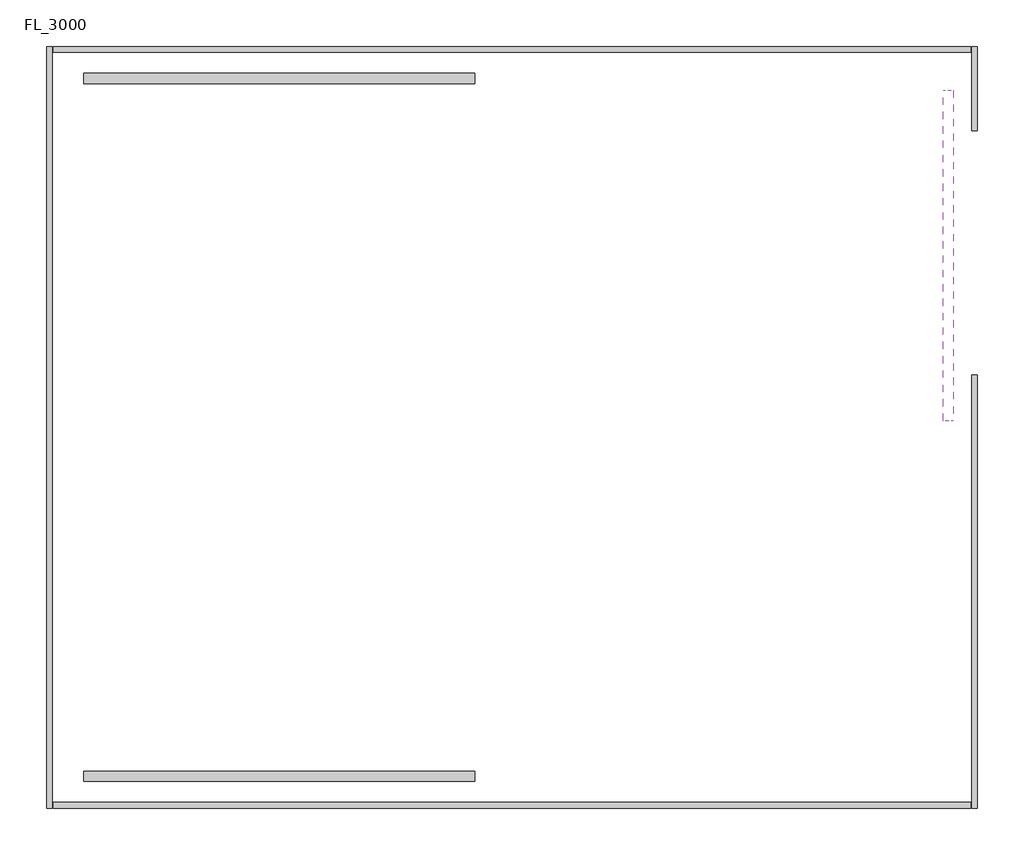
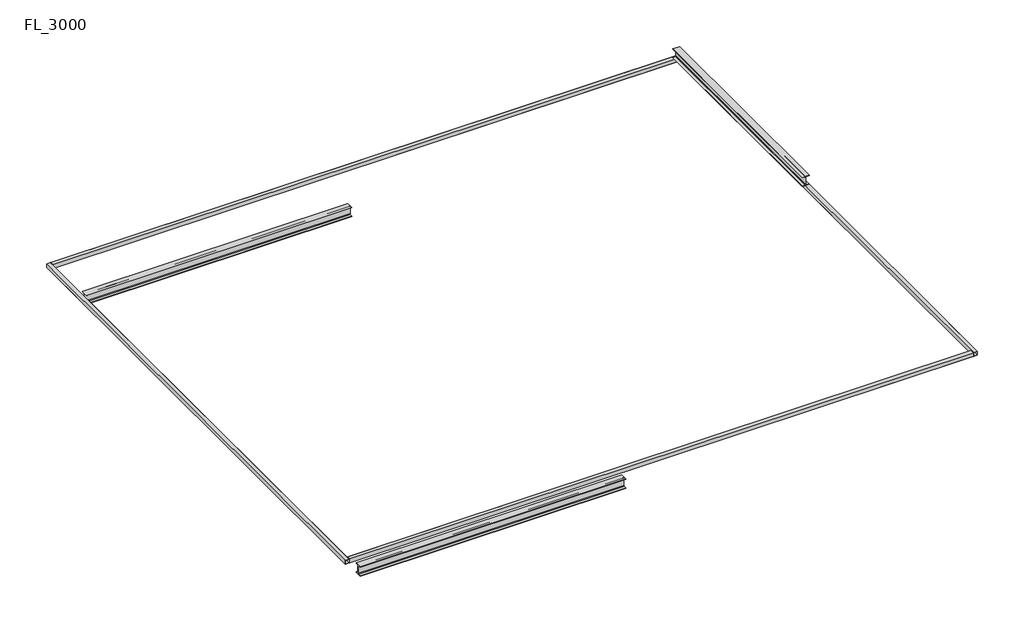
# One storey: 8 beams.
"""IFC4 building model written with IfcOpenShell, lengths in millimetres."""

import ifcopenshell
import ifcopenshell.guid

model = None  # the IFC model being written
_history = None  # IfcOwnerHistory: only IFC2X3 demands one
_inside = {}  # id of a spatial element -> (the spatial element, [elements in it])
_under = {}  # id of a project, library or spatial element -> (it, [spatial elements below it])
_declared = {}  # id of a project -> (the project, [libraries it declares])
_typed = {}  # id of a type object -> (the type object, [elements of that type])
_made_of = {}  # id of a material, layer set ... -> (it, [elements and type objects made of it])


def new_model(schema):
    """Start an empty IFC model of exactly this schema.

    Asked for "IFC4X3", IfcOpenShell would pick the latest addendum, in which some entities
    have other attributes; the version numbers below select the first issue.
    IFC2X3 requires an IfcOwnerHistory on every rooted entity: one is made here for all.
    """
    global model, _history
    if schema == "IFC4X3":
        model = ifcopenshell.file(schema_version=(4, 3, 0, 0))
    else:
        model = ifcopenshell.file(schema=schema)
    _inside.clear()
    _under.clear()
    _declared.clear()
    _typed.clear()
    _made_of.clear()
    _history = None
    if model.schema == "IFC2X3":
        org = make("IfcOrganization", Name="unknown")
        user = make(
            "IfcPersonAndOrganization",
            ThePerson=make("IfcPerson", FamilyName="unknown"),
            TheOrganization=org,
        )
        app = make(
            "IfcApplication",
            ApplicationDeveloper=org,
            Version="unknown",
            ApplicationFullName="unknown",
            ApplicationIdentifier="unknown",
        )
        _history = make(
            "IfcOwnerHistory",
            OwningUser=user,
            OwningApplication=app,
            ChangeAction="ADDED",
            CreationDate=0,
        )
    return model


def make(cls, **values):
    """One entity of the class cls with the attributes given. An attribute that is None is left unset."""
    return model.create_entity(
        cls, **{name: value for name, value in values.items() if value is not None}
    )


def rooted(cls, **values):
    """An entity with a GlobalId (a new one), such as an element, a storey or a relation."""
    return make(cls, GlobalId=ifcopenshell.guid.new(), OwnerHistory=_history, **values)


def si_unit(unit_type, name, prefix=None):
    """IfcSIUnit, for example si_unit("LENGTHUNIT", "METRE", prefix="MILLI")."""
    return make("IfcSIUnit", UnitType=unit_type, Prefix=prefix, Name=name)


def assignment(units):
    """IfcUnitAssignment: the units of a project."""
    return None if units is None else make("IfcUnitAssignment", Units=units)


def point(xyz):
    """IfcCartesianPoint."""
    return None if xyz is None else make("IfcCartesianPoint", Coordinates=xyz)


def direction(xyz):
    """IfcDirection."""
    return None if xyz is None else make("IfcDirection", DirectionRatios=xyz)


def frame(location, z_axis=None, x_axis=None):
    """IfcAxis2Placement3D, a coordinate frame: its origin and axes. An axis left out is left unset."""
    return make(
        "IfcAxis2Placement3D",
        Location=point(location),
        Axis=direction(z_axis),
        RefDirection=direction(x_axis),
    )


def frame_2d(location, x_axis=None):
    """IfcAxis2Placement2D, a coordinate frame in the plane: its origin and x axis."""
    return make(
        "IfcAxis2Placement2D", Location=point(location), RefDirection=direction(x_axis)
    )


def origin():
    """The frame at (0, 0, 0) with its axes left unset."""
    return frame((0.0, 0.0, 0.0))


def place(relative_to, where):
    """IfcLocalPlacement: puts the frame where relative to a parent placement (None: the world)."""
    return make(
        "IfcLocalPlacement", PlacementRelTo=relative_to, RelativePlacement=where
    )


def context(
    kind, dimensions, precision=None, world=None, true_north=None, identifier=None
):
    """IfcGeometricRepresentationContext, for example the 3D "Model" context."""
    return make(
        "IfcGeometricRepresentationContext",
        ContextIdentifier=identifier,
        ContextType=kind,
        CoordinateSpaceDimension=dimensions,
        Precision=precision,
        WorldCoordinateSystem=world,
        TrueNorth=true_north,
    )


def project(units=None, contexts=None):
    """IfcProject with its units and contexts."""
    return rooted(
        "IfcProject",
        Name="project",
        RepresentationContexts=contexts,
        UnitsInContext=assignment(units),
    )


def spatial(cls, under=None, at=None, **own):
    """A site, building, storey or space (cls), placed at a placement, below another one or the project."""
    s = rooted(cls, ObjectPlacement=at, **own)
    if under is not None:
        _under.setdefault(under.id(), (under, []))[1].append(s)
    return s


def polyline(points):
    """IfcPolyline through the points."""
    return make("IfcPolyline", Points=[point(p) for p in points])


def circle_curve(where, radius):
    """IfcCircle in the frame where."""
    return make("IfcCircle", Position=where, Radius=radius)


def trimmed(basis, trim1, trim2, sense, master):
    """IfcTrimmedCurve: the piece of a basis curve between two trims."""
    return make(
        "IfcTrimmedCurve",
        BasisCurve=basis,
        Trim1=trim1,
        Trim2=trim2,
        SenseAgreement=sense,
        MasterRepresentation=master,
    )


def segment(curve, same_sense, transition):
    """IfcCompositeCurveSegment."""
    return make(
        "IfcCompositeCurveSegment",
        Transition=transition,
        SameSense=same_sense,
        ParentCurve=curve,
    )


def composite_curve(segments, self_intersect=None):
    """IfcCompositeCurve: segments joined end to end."""
    return make("IfcCompositeCurve", Segments=segments, SelfIntersect=self_intersect)


def outline(outer, holes=None, kind="AREA"):
    """IfcArbitraryClosedProfileDef: a profile drawn as a closed curve; with holes, ...WithVoids."""
    if holes is None:
        return make("IfcArbitraryClosedProfileDef", ProfileType=kind, OuterCurve=outer)
    return make(
        "IfcArbitraryProfileDefWithVoids",
        ProfileType=kind,
        OuterCurve=outer,
        InnerCurves=holes,
    )


def extrude(swept, where, along, depth):
    """IfcExtrudedAreaSolid: the profile swept, set in the frame where, extruded along a direction by depth."""
    return make(
        "IfcExtrudedAreaSolid",
        SweptArea=swept,
        Position=where,
        ExtrudedDirection=direction(along),
        Depth=depth,
    )


def shape(context_of_items, identifier, shape_type, items):
    """IfcShapeRepresentation: the items that make up one representation, for example the "Body"."""
    return make(
        "IfcShapeRepresentation",
        ContextOfItems=context_of_items,
        RepresentationIdentifier=identifier,
        RepresentationType=shape_type,
        Items=items,
    )


def source(mapping_origin, context_of_items, identifier, shape_type, items):
    """IfcRepresentationMap: a shape defined once, which mapped items show again and again."""
    return make(
        "IfcRepresentationMap",
        MappingOrigin=mapping_origin,
        MappedRepresentation=shape(context_of_items, identifier, shape_type, items),
    )


def transform(
    local_origin,
    x_axis=None,
    y_axis=None,
    z_axis=None,
    scale=None,
    scale2=None,
    scale3=None,
    uniform=True,
):
    """IfcCartesianTransformationOperator3D, or its non-uniform kind. x_axis, y_axis, z_axis: its Axis1, 2, 3."""
    if uniform:
        return make(
            "IfcCartesianTransformationOperator3D",
            Axis1=direction(x_axis),
            Axis2=direction(y_axis),
            LocalOrigin=point(local_origin),
            Scale=scale,
            Axis3=direction(z_axis),
        )
    return make(
        "IfcCartesianTransformationOperator3DnonUniform",
        Axis1=direction(x_axis),
        Axis2=direction(y_axis),
        LocalOrigin=point(local_origin),
        Scale=scale,
        Axis3=direction(z_axis),
        Scale2=scale2,
        Scale3=scale3,
    )


def mapped(mapping_source, mapping_target):
    """IfcMappedItem: shows the shape of a source again, moved by a transform."""
    return make(
        "IfcMappedItem", MappingSource=mapping_source, MappingTarget=mapping_target
    )


def made_of(thing, what):
    """Note that an element or type object is made of a material, layer set ...; save() writes the relation."""
    if what is not None:
        _made_of.setdefault(what.id(), (what, []))[1].append(thing)
    return thing


def element(
    cls,
    number,
    at=None,
    inside=None,
    cuts=None,
    type_object=None,
    material=None,
    context=None,
    identifier="Body",
    shape_type=None,
    held_by="IfcProductDefinitionShape",
    body=None,
    shapes=None,
    **own,
):
    """One element of the class cls, such as IfcWall. Its Tag is "e" and its number.

    at: its placement. inside: the storey or other place that contains it. cuts: it is an
    opening in that element (IfcRelVoidsElement). A single representation is given by context,
    identifier, shape_type and body (its items); several are given by shapes. held_by: the class
    of the entity that holds the representations. save() writes the other relations.
    """
    e = rooted(cls, Tag="e%d" % number, ObjectPlacement=at, **own)
    if body is not None:
        shapes = [shape(context, identifier, shape_type, body)]
    if shapes is not None:
        e.Representation = make(held_by, Representations=shapes)
    if inside is not None:
        _inside.setdefault(inside.id(), (inside, []))[1].append(e)
    if cuts is not None:
        rooted(
            "IfcRelVoidsElement", RelatingBuildingElement=cuts, RelatedOpeningElement=e
        )
    if type_object is not None:
        _typed.setdefault(type_object.id(), (type_object, []))[1].append(e)
    return made_of(e, material)


def aggregate(whole, parts):
    """IfcRelAggregates: a whole, such as a stair, and the parts it consists of."""
    return rooted("IfcRelAggregates", RelatingObject=whole, RelatedObjects=parts)


def save(model, path):
    """Write the relations noted so far, then the file.

    IfcRelAggregates (storeys below a building ...), IfcRelContainedInSpatialStructure (elements
    in a storey), IfcRelDefinesByType, IfcRelAssociatesMaterial and IfcRelDeclares: one each for
    every whole, place, type object, material and project.
    """
    for whole, parts in _under.values():
        aggregate(whole, parts)
    for where, things in _inside.values():
        rooted(
            "IfcRelContainedInSpatialStructure",
            RelatedElements=things,
            RelatingStructure=where,
        )
    for kind, things in _typed.values():
        rooted("IfcRelDefinesByType", RelatedObjects=things, RelatingType=kind)
    for what, things in _made_of.values():
        rooted("IfcRelAssociatesMaterial", RelatedObjects=things, RelatingMaterial=what)
    for by, libraries in _declared.values():
        rooted("IfcRelDeclares", RelatingContext=by, RelatedDefinitions=libraries)
    model.write(path)


def steel_h_beam_22148b76(model_context):
    return source(origin(), model_context, "Body", "SweptSolid", [
        extrude(outline(composite_curve([segment(polyline([(87.5, -111.0), (87.5, -122.0), (-87.5, -122.0), (-87.5, -111.0), (-19.5, -111.0)]), True, "CONTINUOUS"), segment(trimmed(circle_curve(frame_2d((-19.5, -95.0)), 16.0), [point((-19.5, -111.0))], [point((-3.5, -95.0))], True, "CARTESIAN"), True, "CONTINUOUS"), segment(polyline([(-3.5, -95.0), (-3.5, 95.0)]), True, "CONTINUOUS"), segment(trimmed(circle_curve(frame_2d((-19.5, 95.0)), 16.0), [point((-3.5, 95.0))], [point((-19.5, 111.0))], True, "CARTESIAN"), True, "CONTINUOUS"), segment(polyline([(-19.5, 111.0), (-87.5, 111.0), (-87.5, 122.0), (87.5, 122.0), (87.5, 111.0), (19.5, 111.0)]), True, "CONTINUOUS"), segment(trimmed(circle_curve(frame_2d((19.5, 95.0)), 16.0), [point((19.5, 111.0))], [point((3.5, 95.0))], True, "CARTESIAN"), True, "CONTINUOUS"), segment(polyline([(3.5, 95.0), (3.5, -95.0)]), True, "CONTINUOUS"), segment(trimmed(circle_curve(frame_2d((19.5, -95.0)), 16.0), [point((3.5, -95.0))], [point((19.5, -111.0))], True, "CARTESIAN"), True, "CONTINUOUS"), segment(polyline([(19.5, -111.0), (87.5, -111.0)]), True, "CONTINUOUS")], self_intersect=False)), frame((-3361.8243373, 0.0, 0.0), z_axis=(1.0, 0.0, 0.0), x_axis=(0.0, 1.0, 0.0)), (0.0, 0.0, 1.0), 6724.6),
    ])


def steel_h_beam_0520d745(model_context):
    return source(origin(), model_context, "Body", "SweptSolid", [
        extrude(outline(composite_curve([segment(polyline([(87.5, -111.0), (87.5, -122.0), (-87.5, -122.0), (-87.5, -111.0), (-19.5, -111.0)]), True, "CONTINUOUS"), segment(trimmed(circle_curve(frame_2d((-19.5, -95.0)), 16.0), [point((-19.5, -111.0))], [point((-3.5, -95.0))], True, "CARTESIAN"), True, "CONTINUOUS"), segment(polyline([(-3.5, -95.0), (-3.5, 95.0)]), True, "CONTINUOUS"), segment(trimmed(circle_curve(frame_2d((-19.5, 95.0)), 16.0), [point((-3.5, 95.0))], [point((-19.5, 111.0))], True, "CARTESIAN"), True, "CONTINUOUS"), segment(polyline([(-19.5, 111.0), (-87.5, 111.0), (-87.5, 122.0), (87.5, 122.0), (87.5, 111.0), (19.5, 111.0)]), True, "CONTINUOUS"), segment(trimmed(circle_curve(frame_2d((19.5, 95.0)), 16.0), [point((19.5, 111.0))], [point((3.5, 95.0))], True, "CARTESIAN"), True, "CONTINUOUS"), segment(polyline([(3.5, 95.0), (3.5, -95.0)]), True, "CONTINUOUS"), segment(trimmed(circle_curve(frame_2d((19.5, -95.0)), 16.0), [point((3.5, -95.0))], [point((19.5, -111.0))], True, "CARTESIAN"), True, "CONTINUOUS"), segment(polyline([(19.5, -111.0), (87.5, -111.0)]), True, "CONTINUOUS")], self_intersect=False)), frame((-3363.2513255, 0.0, 0.0), z_axis=(1.0, 0.0, 0.0), x_axis=(0.0, 1.0, 0.0)), (0.0, 0.0, 1.0), 6724.6),
    ])


def steel_h_beam_2cee67ca(model_context):
    return source(origin(), model_context, "Body", "SweptSolid", [
        extrude(outline(composite_curve([segment(polyline([(87.5, -111.0), (87.5, -122.0), (-87.5, -122.0), (-87.5, -111.0), (-19.5, -111.0)]), True, "CONTINUOUS"), segment(trimmed(circle_curve(frame_2d((-19.5, -95.0)), 16.0), [point((-19.5, -111.0))], [point((-3.5, -95.0))], True, "CARTESIAN"), True, "CONTINUOUS"), segment(polyline([(-3.5, -95.0), (-3.5, 95.0)]), True, "CONTINUOUS"), segment(trimmed(circle_curve(frame_2d((-19.5, 95.0)), 16.0), [point((-3.5, 95.0))], [point((-19.5, 111.0))], True, "CARTESIAN"), True, "CONTINUOUS"), segment(polyline([(-19.5, 111.0), (-87.5, 111.0), (-87.5, 122.0), (87.5, 122.0), (87.5, 111.0), (19.5, 111.0)]), True, "CONTINUOUS"), segment(trimmed(circle_curve(frame_2d((19.5, 95.0)), 16.0), [point((19.5, 111.0))], [point((3.5, 95.0))], True, "CARTESIAN"), True, "CONTINUOUS"), segment(polyline([(3.5, 95.0), (3.5, -95.0)]), True, "CONTINUOUS"), segment(trimmed(circle_curve(frame_2d((19.5, -95.0)), 16.0), [point((3.5, -95.0))], [point((19.5, -111.0))], True, "CARTESIAN"), True, "CONTINUOUS"), segment(polyline([(19.5, -111.0), (87.5, -111.0)]), True, "CONTINUOUS")], self_intersect=False)), frame((-2886.3486745, 0.0, 0.0), z_axis=(1.0, 0.0, 0.0), x_axis=(0.0, 1.0, 0.0)), (0.0, 0.0, 1.0), 5681.8597388),
    ])


def steel_rectangular_beam_bm125_rt_100x100x4_0_fd47acba(model_context):
    return source(origin(), model_context, "Body", "SweptSolid", [
        extrude(outline(polyline([(-50.0, 50.0), (50.0, 50.0), (50.0, -50.0), (-50.0, -50.0), (-50.0, 50.0)]), holes=[polyline([(46.0, -46.0), (46.0, 46.0), (-46.0, 46.0), (-46.0, -46.0), (46.0, -46.0)])]), frame((-7887.3, 0.0, 0.0), z_axis=(1.0, 0.0, 0.0), x_axis=(0.0, 1.0, 0.0)), (0.0, 0.0, 1.0), 15774.6),
        extrude(outline(polyline([(-50.0, 50.0), (50.0, 50.0), (50.0, -50.0), (-50.0, -50.0), (-50.0, 50.0)]), holes=[polyline([(46.0, -46.0), (46.0, 46.0), (-46.0, 46.0), (-46.0, -46.0), (46.0, -46.0)])]), frame((-7887.3, 0.0, 0.0), z_axis=(1.0, 0.0, 0.0), x_axis=(0.0, 1.0, 0.0)), (0.0, 0.0, 1.0), 15774.6),
        extrude(outline(polyline([(-50.0, 50.0), (50.0, 50.0), (50.0, -50.0), (-50.0, -50.0), (-50.0, 50.0)]), holes=[polyline([(46.0, -46.0), (46.0, 46.0), (-46.0, 46.0), (-46.0, -46.0), (46.0, -46.0)])]), frame((-7887.3, 0.0, 0.0), z_axis=(1.0, 0.0, 0.0), x_axis=(0.0, 1.0, 0.0)), (0.0, 0.0, 1.0), 15774.6),
        extrude(outline(polyline([(-50.0, 50.0), (50.0, 50.0), (50.0, -50.0), (-50.0, -50.0), (-50.0, 50.0)]), holes=[polyline([(46.0, -46.0), (46.0, 46.0), (-46.0, 46.0), (-46.0, -46.0), (46.0, -46.0)])]), frame((-7887.3, 0.0, 0.0), z_axis=(1.0, 0.0, 0.0), x_axis=(0.0, 1.0, 0.0)), (0.0, 0.0, 1.0), 15774.6),
    ])


def steel_rectangular_beam_bm125_rt_100x100x4_0_2c93a6f0(model_context):
    return source(origin(), model_context, "Body", "SweptSolid", [
        extrude(outline(polyline([(-50.0, 50.0), (50.0, 50.0), (50.0, -50.0), (-50.0, -50.0), (-50.0, 50.0)]), holes=[polyline([(46.0, -46.0), (46.0, 46.0), (-46.0, 46.0), (-46.0, -46.0), (46.0, -46.0)])]), frame((-6550.0, 0.0, 0.0), z_axis=(1.0, 0.0, 0.0), x_axis=(0.0, 1.0, 0.0)), (0.0, 0.0, 1.0), 13100.0),
        extrude(outline(polyline([(-50.0, 50.0), (50.0, 50.0), (50.0, -50.0), (-50.0, -50.0), (-50.0, 50.0)]), holes=[polyline([(46.0, -46.0), (46.0, 46.0), (-46.0, 46.0), (-46.0, -46.0), (46.0, -46.0)])]), frame((-6550.0, 0.0, 0.0), z_axis=(1.0, 0.0, 0.0), x_axis=(0.0, 1.0, 0.0)), (0.0, 0.0, 1.0), 13100.0),
        extrude(outline(polyline([(-50.0, 50.0), (50.0, 50.0), (50.0, -50.0), (-50.0, -50.0), (-50.0, 50.0)]), holes=[polyline([(46.0, -46.0), (46.0, 46.0), (-46.0, 46.0), (-46.0, -46.0), (46.0, -46.0)])]), frame((-6550.0, 0.0, 0.0), z_axis=(1.0, 0.0, 0.0), x_axis=(0.0, 1.0, 0.0)), (0.0, 0.0, 1.0), 13100.0),
        extrude(outline(polyline([(-50.0, 50.0), (50.0, 50.0), (50.0, -50.0), (-50.0, -50.0), (-50.0, 50.0)]), holes=[polyline([(46.0, -46.0), (46.0, 46.0), (-46.0, 46.0), (-46.0, -46.0), (46.0, -46.0)])]), frame((-6550.0, 0.0, 0.0), z_axis=(1.0, 0.0, 0.0), x_axis=(0.0, 1.0, 0.0)), (0.0, 0.0, 1.0), 13100.0),
    ])


def steel_rectangular_beam_bm125_rt_100x100x4_0_60a5dd41(model_context):
    return source(origin(), model_context, "Body", "SweptSolid", [
        extrude(outline(polyline([(-50.0, 50.0), (50.0, 50.0), (50.0, -50.0), (-50.0, -50.0), (-50.0, 50.0)]), holes=[polyline([(46.0, -46.0), (46.0, 46.0), (-46.0, 46.0), (-46.0, -46.0), (46.0, -46.0)])]), frame((-3725.0, 0.0, 0.0), z_axis=(1.0, 0.0, 0.0), x_axis=(0.0, 1.0, 0.0)), (0.0, 0.0, 1.0), 7450.0),
        extrude(outline(polyline([(-50.0, 50.0), (50.0, 50.0), (50.0, -50.0), (-50.0, -50.0), (-50.0, 50.0)]), holes=[polyline([(46.0, -46.0), (46.0, 46.0), (-46.0, 46.0), (-46.0, -46.0), (46.0, -46.0)])]), frame((-3725.0, 0.0, 0.0), z_axis=(1.0, 0.0, 0.0), x_axis=(0.0, 1.0, 0.0)), (0.0, 0.0, 1.0), 7450.0),
        extrude(outline(polyline([(-50.0, 50.0), (50.0, 50.0), (50.0, -50.0), (-50.0, -50.0), (-50.0, 50.0)]), holes=[polyline([(46.0, -46.0), (46.0, 46.0), (-46.0, 46.0), (-46.0, -46.0), (46.0, -46.0)])]), frame((-3725.0, 0.0, 0.0), z_axis=(1.0, 0.0, 0.0), x_axis=(0.0, 1.0, 0.0)), (0.0, 0.0, 1.0), 7450.0),
        extrude(outline(polyline([(-50.0, 50.0), (50.0, 50.0), (50.0, -50.0), (-50.0, -50.0), (-50.0, 50.0)]), holes=[polyline([(46.0, -46.0), (46.0, 46.0), (-46.0, 46.0), (-46.0, -46.0), (46.0, -46.0)])]), frame((-3725.0, 0.0, 0.0), z_axis=(1.0, 0.0, 0.0), x_axis=(0.0, 1.0, 0.0)), (0.0, 0.0, 1.0), 7450.0),
    ])


def steel_rectangular_beam_bm125_rt_100x100x4_0_366960fc(model_context):
    return source(origin(), model_context, "Body", "SweptSolid", [
        extrude(outline(polyline([(-50.0, 50.0), (50.0, 50.0), (50.0, -50.0), (-50.0, -50.0), (-50.0, 50.0)]), holes=[polyline([(46.0, -46.0), (46.0, 46.0), (-46.0, 46.0), (-46.0, -46.0), (46.0, -46.0)])]), frame((-725.0, 0.0, 0.0), z_axis=(1.0, 0.0, 0.0), x_axis=(0.0, 1.0, 0.0)), (0.0, 0.0, 1.0), 1450.0),
        extrude(outline(polyline([(-50.0, 50.0), (50.0, 50.0), (50.0, -50.0), (-50.0, -50.0), (-50.0, 50.0)]), holes=[polyline([(46.0, -46.0), (46.0, 46.0), (-46.0, 46.0), (-46.0, -46.0), (46.0, -46.0)])]), frame((-725.0, 0.0, 0.0), z_axis=(1.0, 0.0, 0.0), x_axis=(0.0, 1.0, 0.0)), (0.0, 0.0, 1.0), 1450.0),
        extrude(outline(polyline([(-50.0, 50.0), (50.0, 50.0), (50.0, -50.0), (-50.0, -50.0), (-50.0, 50.0)]), holes=[polyline([(46.0, -46.0), (46.0, 46.0), (-46.0, 46.0), (-46.0, -46.0), (46.0, -46.0)])]), frame((-725.0, 0.0, 0.0), z_axis=(1.0, 0.0, 0.0), x_axis=(0.0, 1.0, 0.0)), (0.0, 0.0, 1.0), 1450.0),
        extrude(outline(polyline([(-50.0, 50.0), (50.0, 50.0), (50.0, -50.0), (-50.0, -50.0), (-50.0, 50.0)]), holes=[polyline([(46.0, -46.0), (46.0, 46.0), (-46.0, 46.0), (-46.0, -46.0), (46.0, -46.0)])]), frame((-725.0, 0.0, 0.0), z_axis=(1.0, 0.0, 0.0), x_axis=(0.0, 1.0, 0.0)), (0.0, 0.0, 1.0), 1450.0),
    ])


model = new_model("IFC4")

# Units and contexts
model_context = context("Model", 3, world=origin())
ifc_project = project(units=[si_unit("LENGTHUNIT", "METRE", prefix="MILLI")], contexts=[model_context])

# Site, building, storey
site = spatial("IfcSite", under=ifc_project)
building = spatial("IfcBuilding", under=site)
storey = spatial("IfcBuildingStorey", under=building, Name="FL_3000", Elevation=3000.0)

# Beams
placement = place(None, origin())
steel_h_beam_shape = steel_h_beam_22148b76(model_context)
element("IfcBeam", 1, ObjectType="Steel-H-Beam : BM121_H-244×175x7x11", at=placement, inside=storey, context=model_context, shape_type="MappedRepresentation", body=[
    mapped(steel_h_beam_shape, transform((2100.4756627, 10594.5382614, 3000.0), x_axis=(1.0, 0.0, 0.0), y_axis=(0.0, 1.0, 0.0), z_axis=(0.0, 0.0, 1.0))),
])
steel_h_beam_2_shape = steel_h_beam_0520d745(model_context)
element("IfcBeam", 2, ObjectType="Steel-H-Beam : BM121_H-244×175x7x11", at=placement, inside=storey, context=model_context, shape_type="MappedRepresentation", body=[
    mapped(steel_h_beam_2_shape, transform((2100.0, 22594.5382614, 3000.0), x_axis=(-1.0, 0.0, 0.0), y_axis=(0.0, -1.0, 0.0), z_axis=(0.0, 0.0, 1.0))),
])
steel_h_beam_3_shape = steel_h_beam_2cee67ca(model_context)
element("IfcBeam", 3, ObjectType="Steel-H-Beam : BM121_H-244×175x7x11", at=placement, inside=storey, context=model_context, shape_type="MappedRepresentation", body=[
    mapped(steel_h_beam_3_shape, transform((13600.0, 19594.5382614, 4500.0), x_axis=(0.0, 1.0, 0.0), y_axis=(-1.0, 0.0, 0.0), z_axis=(0.0, 0.0, 1.0))),
])
steel_rectangular_beam_bm125_rt_100x100x4_0_shape = steel_rectangular_beam_bm125_rt_100x100x4_0_fd47acba(model_context)
element("IfcBeam", 4, ObjectType="Steel-Rectangular-Beam : BM125_RT-100x100x4.0", at=placement, inside=storey, context=model_context, shape_type="MappedRepresentation", body=[
    mapped(steel_rectangular_beam_bm125_rt_100x100x4_0_shape, transform((6100.0, 10094.5382614, 3750.0), x_axis=(1.0, 0.0, 0.0), y_axis=(0.0, 1.0, 0.0), z_axis=(0.0, 0.0, 1.0))),
])
element("IfcBeam", 5, ObjectType="Steel-Rectangular-Beam : BM125_RT-100x100x4.0", at=placement, inside=storey, context=model_context, shape_type="MappedRepresentation", body=[
    mapped(steel_rectangular_beam_bm125_rt_100x100x4_0_shape, transform((6100.0, 23094.5382614, 3750.0), x_axis=(-1.0, 0.0, 0.0), y_axis=(0.0, -1.0, 0.0), z_axis=(0.0, 0.0, 1.0))),
])
steel_rectangular_beam_bm125_rt_100x100x4_0_2_shape = steel_rectangular_beam_bm125_rt_100x100x4_0_2c93a6f0(model_context)
element("IfcBeam", 6, ObjectType="Steel-Rectangular-Beam : BM125_RT-100x100x4.0", at=placement, inside=storey, context=model_context, shape_type="MappedRepresentation", body=[
    mapped(steel_rectangular_beam_bm125_rt_100x100x4_0_2_shape, transform((-1850.0, 16594.5382614, 3750.0), x_axis=(0.0, -1.0, 0.0), y_axis=(1.0, 0.0, 0.0), z_axis=(0.0, 0.0, 1.0))),
])
steel_rectangular_beam_bm125_rt_100x100x4_0_3_shape = steel_rectangular_beam_bm125_rt_100x100x4_0_60a5dd41(model_context)
element("IfcBeam", 7, ObjectType="Steel-Rectangular-Beam : BM125_RT-100x100x4.0", at=placement, inside=storey, context=model_context, shape_type="MappedRepresentation", body=[
    mapped(steel_rectangular_beam_bm125_rt_100x100x4_0_3_shape, transform((14050.0, 13769.5382614, 3750.0), x_axis=(0.0, 1.0, 0.0), y_axis=(-1.0, 0.0, 0.0), z_axis=(0.0, 0.0, 1.0))),
])
steel_rectangular_beam_bm125_rt_100x100x4_0_4_shape = steel_rectangular_beam_bm125_rt_100x100x4_0_366960fc(model_context)
element("IfcBeam", 8, ObjectType="Steel-Rectangular-Beam : BM125_RT-100x100x4.0", at=placement, inside=storey, context=model_context, shape_type="MappedRepresentation", body=[
    mapped(steel_rectangular_beam_bm125_rt_100x100x4_0_4_shape, transform((14050.0, 22419.5382614, 3750.0), x_axis=(0.0, 1.0, 0.0), y_axis=(-1.0, 0.0, 0.0), z_axis=(0.0, 0.0, 1.0))),
])

save(model, "model.ifc")

# Revit data of these elements
# Type "Steel-H-Beam : BM121_H-244×175x7x11"
#   Surface Area = 0.00 m²/m
#   Section Area = 56.24 cm²
#   Mass per Unit Length = 44.10 kg/m
#   Length [instance default] = 1524 mm
#   B = 175 mm
#   H = 244 mm
#   r = 16 mm
#   tw = 7 mm
#   tf = 11 mm
#   hec_material4 [instance default] = none
#   hec_material3 [instance default] = none
#   hec_material2 [instance default] = none
#   hec_material1 [instance default] = none
#   Structural Material [instance default] = Steel, 45-345
#   Assembly Code = ""
# Type "Steel-Rectangular-Beam : BM125_RT-100x100x4.0"
#   t = 4 mm
#   Mass per Unit Length = 11.70 kg/m
#   Surface Area = 0.386 m²/m
#   Sectional Area = 14.95 cm²
#   Length [instance default] = 3000 mm
#   H = 100 mm
#   B = 100 mm
#   hec_material4 [instance default] = none
#   hec_material3 [instance default] = none
#   hec_material2 [instance default] = none
#   hec_material1 [instance default] = none
#   Structural Material [instance default] = none
# Elements 1, 2, 3 (IfcBeam, "Steel-H-Beam : BM121_H-244×175x7x11")
#   Comments = ""
#   F01) Building Name = "Fire Water Pump Building"
#   F11) Project Building Tag_Type-1 = ""
#   F12) Project Building Tag_Type-2 = ""
#   F13) Project Facility Code = "621"
#   F21) Structural Type = "Steel"
#   F31) Standard Building Code = "E204"
#   F41) Discipline = "Architecture"
#   F51) Plan Start Date-Engineering = "2018-09-14"
#   F52) Plan Finish Date-Engineering = "2019-12-02"
#   F53) Duration = "444"
#   W11) Activity ID = "T3C621AR4110"
#   W12) Activity Name = "Fire Water Pump BLDG - Main Steel Structure"
#   W13) Plan Start Date = "2019-04-02"
#   W14) Plan Finish Date = "2019-06-03"
#   Structural Material = S01AA002-00001_Main Steel Structure Fabrication Work_Shelter/Building_Medium Steel - Standard
#   hec_material4 = S01AA010-00002_Main Steel Structure Fabrication Work_Shelter/Building_Steel Painting/Coating_for Fireproofed Steel Surface, Surface Preparation & Primer Coat
#   hec_material3 = F01AC000-00002_Building/Shelter Fire Proofing Work_Intumescent Coating Type_1 hr. rating (UL 1709))
#   hec_material2 = S01AA010-00001_Main Steel Structure Fabrication Work_Shelter/Building_Steel Painting/Coating_for Non-Fireproofed Steel Surface, Surface Preparation, Primer, Second & Final Coat
#   hec_material1 = S03AA028-00001_Main Steel Structure Erection Work_Shelter/Building_Medium Steel
#   Phase Created = New Construction
#   Materials on its faces: "Steel, 45-345"
# Elements 4, 5, 6, 7, 8 (IfcBeam, "Steel-Rectangular-Beam : BM125_RT-100x100x4.0")
#   Comments = ""
#   F01) Building Name = "Fire Water Pump Building"
#   F11) Project Building Tag_Type-1 = ""
#   F12) Project Building Tag_Type-2 = ""
#   F13) Project Facility Code = "621"
#   F21) Structural Type = "Steel"
#   F31) Standard Building Code = "E204"
#   F41) Discipline = "Architecture"
#   F51) Plan Start Date-Engineering = "2018-09-14"
#   F52) Plan Finish Date-Engineering = "2019-12-02"
#   F53) Duration = "444"
#   W11) Activity ID = "T3C621AR4110"
#   W12) Activity Name = "Fire Water Pump BLDG - Main Steel Structure"
#   W13) Plan Start Date = "2019-04-02"
#   W14) Plan Finish Date = "2019-06-03"
#   hec_material4 = none
#   hec_material3 = none
#   hec_material2 = S01AA010-00001_Main Steel Structure Fabrication Work_Shelter/Building_Steel Painting/Coating_for Non-Fireproofed Steel Surface, Surface Preparation, Primer, Second & Final Coat
#   hec_material1 = S03AA007-00001_Main Steel Structure Erection Work_Girth & Purlin
#   Structural Material = S01AA007-00001_Main Steel Structure Fabrication Work_Shelter/Building_Girth & Purlin
#   Phase Created = New Construction
#   Materials on its faces: "S01AA010-00001_Main Steel Structure Fabrication Work_Shelter/Building_Steel Painting/Coating_for Non-Fireproofed Steel Surface, Surface Preparation, Primer, Second & Final Coat"
# Materials
#   "Steel, 45-345": class "Metal", colour RGB 189 187 185, transparency 0, Description = "Steel 345 MPa", Cost = 0
#   "S01AA002-00001_Main Steel Structure Fabrication Work_Shelter/Building_Medium Steel - Standard": class "Metal", colour RGB 120 120 120, transparency 0, Comments = "(90KG/M>Weight≥30KG/M)", Description = "Structural steel 50ksi", W00) Work Master Code = "S01AA002-0001", W01) Work Master_Lv1 = "Main Steel Structure Fabrication Work", W02) Work Master_Lv2 = "Shelter/Building", W03) Work Master_Spec.1 = "Medium Steel - Standard (90KG/M>Weight≥30KG/M)", Cost = 0
#   "S01AA010-00002_Main Steel Structure Fabrication Work_Shelter/Building_Steel Painting/Coating_for Fireproofed Steel Surface, Surface Preparation & Primer Coat": class "Metal", colour RGB 120 120 120, transparency 0, Description = "Paint finished steel", W00) Work Master Code = "SS01AA010-00002", W01) Work Master_Lv1 = "Main Steel Structure Fabrication Work", W02) Work Master_Lv2 = "Shelter/Building", W03) Work Master_Spec.1 = "Steel Painting/Coating", W04) Work Master_Spec.2 = "for Fireproofed Steel Surface, Surface Preparation & Primer Coat", Cost = 0
#   "F01AC000-00002_Building/Shelter Fire Proofing Work_Intumescent Coating Type_1 hr. rating (UL 1709))": class "Metal", colour RGB 255 128 128, transparency 0, Description = "Paint finished steel", W00) Work Master Code = "F01AC000-00002", W01) Work Master_Lv1 = "Building/Shelter Fire Proofing Work", W02) Work Master_Lv2 = "Intumescent Coating Type", W03) Work Master_Spec.1 = "1 hr. rating (UL 1709)", Cost = 0
#   "S01AA010-00001_Main Steel Structure Fabrication Work_Shelter/Building_Steel Painting/Coating_for Non-Fireproofed Steel Surface, Surface Preparation, Primer, Second & Final Coat": class "Metal", colour RGB 120 120 120, transparency 0, Description = "Paint finished steel", W00) Work Master Code = "S01AA010-00001", W01) Work Master_Lv1 = "Main Steel Structure Fabrication Work", W02) Work Master_Lv2 = "Shelter/Building", W03) Work Master_Spec.1 = "Steel Painting/Coating", W04) Work Master_Spec.2 = "for Non-Fireproofed Steel Surface, Surface Preparation, Primer, Second & Final Coat", Cost = 0
#   "S03AA028-00001_Main Steel Structure Erection Work_Shelter/Building_Medium Steel": class "Metal", colour RGB 120 120 120, transparency 0, Comments = "(90KG/M>Weight≥30KG/M)", Description = "Structural steel 50ksi", W00) Work Master Code = "S03AA028-0001", W01) Work Master_Lv1 = "Main Steel Structure Erection Work", W02) Work Master_Lv2 = "Shelter/Building", W03) Work Master_Spec.1 = "Medium Steel (90KG/M>Weight≥30KG/M)", Cost = 0
#   "S03AA007-00001_Main Steel Structure Erection Work_Girth & Purlin": class "Metal", colour RGB 120 120 120, transparency 0, Comments = "(30KG/M>Weight)", Description = "Structural steel 50ksi", W00) Work Master Code = "S03AA007-00001", W01) Work Master_Lv1 = "Main Steel Structure Erection Work", W02) Work Master_Lv2 = "Shelter/Building", W03) Work Master_Spec.1 = "Girth & Purlin", Cost = 0
#   "S01AA007-00001_Main Steel Structure Fabrication Work_Shelter/Building_Girth & Purlin": class "Metal", colour RGB 120 120 120, transparency 0, Comments = "(30KG/M>Weight)", Description = "Structural steel 50ksi", W00) Work Master Code = "S01AA007-00001", W01) Work Master_Lv1 = "Main Steel Structure Fabrication Work", W02) Work Master_Lv2 = "Shelter/Building", W03) Work Master_Spec.1 = "Girth & Purlin", Cost = 0
